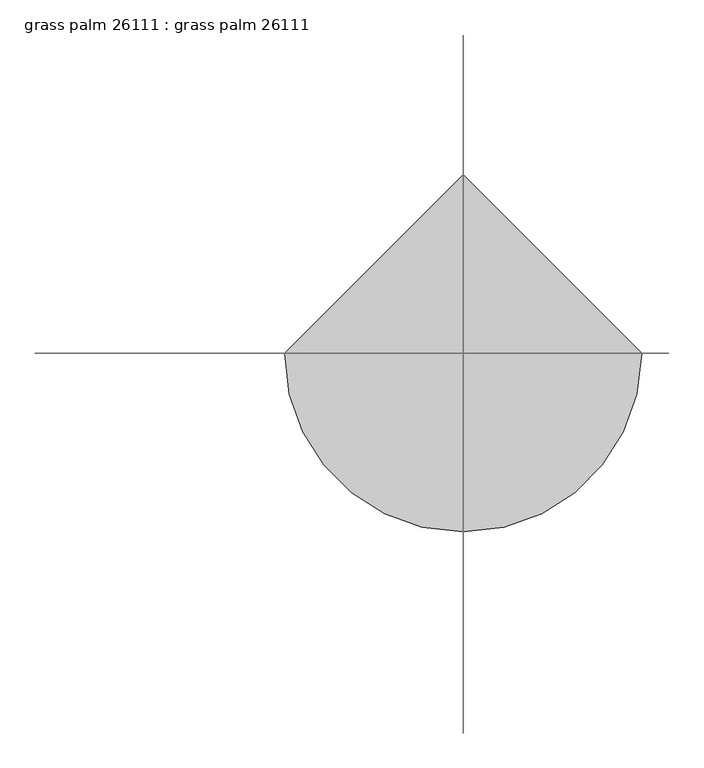
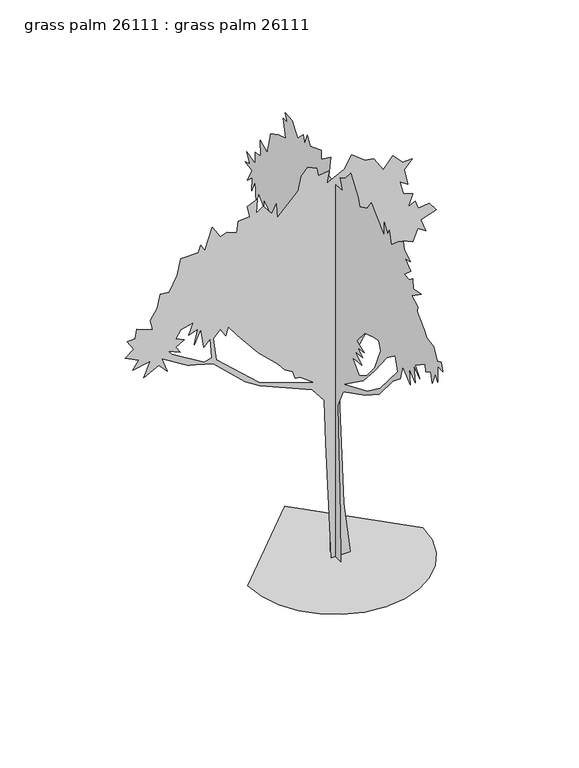
"""IFC4 building model written with IfcOpenShell, lengths in millimetres: proxy geometry, grass palm 26111 : grass palm 26111."""

import ifcopenshell
import ifcopenshell.guid

model = None  # the IFC model being written
_history = None  # IfcOwnerHistory: only IFC2X3 demands one
_inside = {}  # id of a spatial element -> (the spatial element, [elements in it])
_under = {}  # id of a project, library or spatial element -> (it, [spatial elements below it])
_declared = {}  # id of a project -> (the project, [libraries it declares])
_typed = {}  # id of a type object -> (the type object, [elements of that type])
_made_of = {}  # id of a material, layer set ... -> (it, [elements and type objects made of it])


def new_model(schema):
    """Start an empty IFC model of exactly this schema.

    Asked for "IFC4X3", IfcOpenShell would pick the latest addendum, in which some entities
    have other attributes; the version numbers below select the first issue.
    IFC2X3 requires an IfcOwnerHistory on every rooted entity: one is made here for all.
    """
    global model, _history
    if schema == "IFC4X3":
        model = ifcopenshell.file(schema_version=(4, 3, 0, 0))
    else:
        model = ifcopenshell.file(schema=schema)
    _inside.clear()
    _under.clear()
    _declared.clear()
    _typed.clear()
    _made_of.clear()
    _history = None
    if model.schema == "IFC2X3":
        org = make("IfcOrganization", Name="unknown")
        user = make(
            "IfcPersonAndOrganization",
            ThePerson=make("IfcPerson", FamilyName="unknown"),
            TheOrganization=org,
        )
        app = make(
            "IfcApplication",
            ApplicationDeveloper=org,
            Version="unknown",
            ApplicationFullName="unknown",
            ApplicationIdentifier="unknown",
        )
        _history = make(
            "IfcOwnerHistory",
            OwningUser=user,
            OwningApplication=app,
            ChangeAction="ADDED",
            CreationDate=0,
        )
    return model


def make(cls, **values):
    """One entity of the class cls with the attributes given. An attribute that is None is left unset."""
    return model.create_entity(
        cls, **{name: value for name, value in values.items() if value is not None}
    )


def rooted(cls, **values):
    """An entity with a GlobalId (a new one), such as an element, a storey or a relation."""
    return make(cls, GlobalId=ifcopenshell.guid.new(), OwnerHistory=_history, **values)


def si_unit(unit_type, name, prefix=None):
    """IfcSIUnit, for example si_unit("LENGTHUNIT", "METRE", prefix="MILLI")."""
    return make("IfcSIUnit", UnitType=unit_type, Prefix=prefix, Name=name)


def assignment(units):
    """IfcUnitAssignment: the units of a project."""
    return None if units is None else make("IfcUnitAssignment", Units=units)


def point(xyz):
    """IfcCartesianPoint."""
    return None if xyz is None else make("IfcCartesianPoint", Coordinates=xyz)


def direction(xyz):
    """IfcDirection."""
    return None if xyz is None else make("IfcDirection", DirectionRatios=xyz)


def frame(location, z_axis=None, x_axis=None):
    """IfcAxis2Placement3D, a coordinate frame: its origin and axes. An axis left out is left unset."""
    return make(
        "IfcAxis2Placement3D",
        Location=point(location),
        Axis=direction(z_axis),
        RefDirection=direction(x_axis),
    )


def origin():
    """The frame at (0, 0, 0) with its axes left unset."""
    return frame((0.0, 0.0, 0.0))


def place(relative_to, where):
    """IfcLocalPlacement: puts the frame where relative to a parent placement (None: the world)."""
    return make(
        "IfcLocalPlacement", PlacementRelTo=relative_to, RelativePlacement=where
    )


def context(
    kind, dimensions, precision=None, world=None, true_north=None, identifier=None
):
    """IfcGeometricRepresentationContext, for example the 3D "Model" context."""
    return make(
        "IfcGeometricRepresentationContext",
        ContextIdentifier=identifier,
        ContextType=kind,
        CoordinateSpaceDimension=dimensions,
        Precision=precision,
        WorldCoordinateSystem=world,
        TrueNorth=true_north,
    )


def project(units=None, contexts=None):
    """IfcProject with its units and contexts."""
    return rooted(
        "IfcProject",
        Name="project",
        RepresentationContexts=contexts,
        UnitsInContext=assignment(units),
    )


def spatial(cls, under=None, at=None, **own):
    """A site, building, storey or space (cls), placed at a placement, below another one or the project."""
    s = rooted(cls, ObjectPlacement=at, **own)
    if under is not None:
        _under.setdefault(under.id(), (under, []))[1].append(s)
    return s


def point_list(points):
    """IfcCartesianPointList2D or 3D."""
    cls = (
        "IfcCartesianPointList2D" if len(points[0]) == 2 else "IfcCartesianPointList3D"
    )
    return make(cls, CoordList=points)


def triangles(points, corners, closed=None, point_numbers=None):
    """IfcTriangulatedFaceSet: each triangle names its three corners, points numbered from 1."""
    return make(
        "IfcTriangulatedFaceSet",
        Coordinates=point_list(points),
        Closed=closed,
        CoordIndex=corners,
        PnIndex=point_numbers,
    )


def shape(context_of_items, identifier, shape_type, items):
    """IfcShapeRepresentation: the items that make up one representation, for example the "Body"."""
    return make(
        "IfcShapeRepresentation",
        ContextOfItems=context_of_items,
        RepresentationIdentifier=identifier,
        RepresentationType=shape_type,
        Items=items,
    )


def source(mapping_origin, context_of_items, identifier, shape_type, items):
    """IfcRepresentationMap: a shape defined once, which mapped items show again and again."""
    return make(
        "IfcRepresentationMap",
        MappingOrigin=mapping_origin,
        MappedRepresentation=shape(context_of_items, identifier, shape_type, items),
    )


def transform(
    local_origin,
    x_axis=None,
    y_axis=None,
    z_axis=None,
    scale=None,
    scale2=None,
    scale3=None,
    uniform=True,
):
    """IfcCartesianTransformationOperator3D, or its non-uniform kind. x_axis, y_axis, z_axis: its Axis1, 2, 3."""
    if uniform:
        return make(
            "IfcCartesianTransformationOperator3D",
            Axis1=direction(x_axis),
            Axis2=direction(y_axis),
            LocalOrigin=point(local_origin),
            Scale=scale,
            Axis3=direction(z_axis),
        )
    return make(
        "IfcCartesianTransformationOperator3DnonUniform",
        Axis1=direction(x_axis),
        Axis2=direction(y_axis),
        LocalOrigin=point(local_origin),
        Scale=scale,
        Axis3=direction(z_axis),
        Scale2=scale2,
        Scale3=scale3,
    )


def mapped(mapping_source, mapping_target):
    """IfcMappedItem: shows the shape of a source again, moved by a transform."""
    return make(
        "IfcMappedItem", MappingSource=mapping_source, MappingTarget=mapping_target
    )


def made_of(thing, what):
    """Note that an element or type object is made of a material, layer set ...; save() writes the relation."""
    if what is not None:
        _made_of.setdefault(what.id(), (what, []))[1].append(thing)
    return thing


def element(
    cls,
    number,
    at=None,
    inside=None,
    cuts=None,
    type_object=None,
    material=None,
    context=None,
    identifier="Body",
    shape_type=None,
    held_by="IfcProductDefinitionShape",
    body=None,
    shapes=None,
    **own,
):
    """One element of the class cls, such as IfcWall. Its Tag is "e" and its number.

    at: its placement. inside: the storey or other place that contains it. cuts: it is an
    opening in that element (IfcRelVoidsElement). A single representation is given by context,
    identifier, shape_type and body (its items); several are given by shapes. held_by: the class
    of the entity that holds the representations. save() writes the other relations.
    """
    e = rooted(cls, Tag="e%d" % number, ObjectPlacement=at, **own)
    if body is not None:
        shapes = [shape(context, identifier, shape_type, body)]
    if shapes is not None:
        e.Representation = make(held_by, Representations=shapes)
    if inside is not None:
        _inside.setdefault(inside.id(), (inside, []))[1].append(e)
    if cuts is not None:
        rooted(
            "IfcRelVoidsElement", RelatingBuildingElement=cuts, RelatedOpeningElement=e
        )
    if type_object is not None:
        _typed.setdefault(type_object.id(), (type_object, []))[1].append(e)
    return made_of(e, material)


def aggregate(whole, parts):
    """IfcRelAggregates: a whole, such as a stair, and the parts it consists of."""
    return rooted("IfcRelAggregates", RelatingObject=whole, RelatedObjects=parts)


def save(model, path):
    """Write the relations noted so far, then the file.

    IfcRelAggregates (storeys below a building ...), IfcRelContainedInSpatialStructure (elements
    in a storey), IfcRelDefinesByType, IfcRelAssociatesMaterial and IfcRelDeclares: one each for
    every whole, place, type object, material and project.
    """
    for whole, parts in _under.values():
        aggregate(whole, parts)
    for where, things in _inside.values():
        rooted(
            "IfcRelContainedInSpatialStructure",
            RelatedElements=things,
            RelatingStructure=where,
        )
    for kind, things in _typed.values():
        rooted("IfcRelDefinesByType", RelatedObjects=things, RelatingType=kind)
    for what, things in _made_of.values():
        rooted("IfcRelAssociatesMaterial", RelatedObjects=things, RelatingMaterial=what)
    for by, libraries in _declared.values():
        rooted("IfcRelDeclares", RelatingContext=by, RelatedDefinitions=libraries)
    model.write(path)


def grass_palm_26111_grass_palm_26111_ffc4a38a(model_context):
    return source(origin(), model_context, "Body", "Tessellation", [
        triangles([(197.8251161, -0.0004657, 0.0001367), (109.1148514, -0.0002635, 694.5605118), (43.5490633, 0.0002048, 2380.5060047), (409.1686295, 0.0003079, 2962.5546341), (570.4154732, 0.000405, 3409.2137077), (607.6747178, 0.0004576, 3623.4372597), (719.4525244, 0.0004509, 3660.6992294), (654.2481468, 0.0004936, 3781.8063721), (747.397621, 0.0005252, 3949.4717194), (775.3401741, 0.0005007, 3874.9480705), (877.80376, 0.0005308, 4042.6134178), (1008.2098989, 0.0004934, 3977.4115837), (1073.4142765, 0.0005291, 4145.0772217), (1175.8753189, 0.0004934, 4070.5535728), (1110.6734848, 0.0005514, 4247.5407349), (1315.5981857, 0.0005381, 4312.742569), (1222.4487843, 0.0005851, 4433.8244225), (1082.7284609, 0.0006012, 4415.2060822), (1039.2334414, 0.0006388, 4529.6586891), (952.3222492, 0.0006386, 4480.4079163), (1008.2098989, 0.0006732, 4638.7514488), (886.9528381, 0.0007051, 4688.7640938), (840.544479, 0.0007593, 4862.3223953), (943.0055214, 0.0007261, 4797.0952721), (896.4321287, 0.0007914, 5011.3441132), (998.8957146, 0.0008063, 5123.1297318), (877.80376, 0.0008246, 5123.1297318), (747.397621, 0.0008797, 5253.5334), (626.3056664, 0.0008575, 5104.4861023), (503.8725509, 0.0009294, 5301.1072403), (384.1216845, 0.0009523, 5318.7352341), (216.4545022, 0.0010156, 5458.4604263), (113.9921609, 0.0009855, 5290.795079), (-109.5623986, 0.0009889, 5179.0094604), (-81.6183375, 0.0010277, 5337.3532837), (-221.3396873, 0.0010437, 5318.7352341), (-239.9693097, 0.0010769, 5430.5202713), (-361.0610281, 0.0011104, 5486.4005814), (-444.8937381, 0.0010978, 5393.2585922), (-482.1529827, 0.0010527, 5206.9496155), (-752.2819885, 0.0010175, 4927.5242294), (-770.9103573, 0.0010735, 5123.1297318), (-826.8005505, 0.0010516, 5011.3441132), (-938.5783207, 0.0011065, 5151.0698868), (-1031.7252514, 0.0011028, 5085.8680527), (-1013.0943392, 0.0011506, 5272.1514496), (-1143.5030216, 0.0011551, 5216.2711395), (-1115.557925, 0.0011104, 5067.2244232), (-1264.5950489, 0.0011304, 5057.9278976), (-1283.2232723, 0.0010926, 4908.8806), (-1404.3152996, 0.0011236, 4955.4643845), (-1497.4622303, 0.0011301, 4927.5242294), (-1599.9257435, 0.0011911, 5095.1895767), (-1702.389402, 0.0011281, 4806.4170868), (-1748.9628674, 0.0011604, 4899.5590759), (-1786.2220757, 0.0011407, 4806.4170868), (-2009.7751453, 0.0011745, 4806.4170868), (-2056.3486107, 0.0011233, 4592.1932442), (-2158.8122692, 0.0010856, 4396.5624527), (-2279.9041512, 0.0011064, 4405.8842674), (-2317.1635048, 0.0010639, 4228.8971054), (-2410.3102901, 0.00104, 4089.1972023), (-2377.0008408, 0.0009991, 3957.4473953), (-2587.2949814, 0.0010515, 4033.2916031), (-2605.9133217, 0.0010214, 3912.2100403), (-2708.3768349, 0.0010343, 3902.8882256), (-2624.5569511, 0.0009862, 3772.4845573), (-2736.3166992, 0.0009803, 3688.6390938), (-2559.355117, 0.0009282, 3595.4973953), (-2633.853186, 0.0009091, 3483.7117767), (-2410.3102901, 0.000888, 3530.2955612), (-2494.1431091, 0.0008475, 3334.6900589), (-2298.535136, 0.0008458, 3437.1535721), (-2186.7573658, 0.000796, 3316.0464294), (-2261.2733116, 0.0008604, 3511.6772209), (-1928.0074619, 0.0007539, 3305.1500015), (-1586.5374619, 0.000677, 3211.8556961), (-1169.4034029, 0.0005069, 2817.7745178), (-980.3029541, 0.0004448, 2694.5084953), (-299.9587802, 0.0002625, 2401.7378483), (-143.374379, 0.000185, 2203.9150394), (-126.1084725, 2.08e-05, 1609.6107628), (-53.6737587, -0.0004278, 0.0001367), (-1497.4622303, 0.0008957, 3651.4027039), (-1422.9462845, 0.000854, 3539.6173759), (-1395.0011879, 0.0008802, 3651.4027039), (-1273.9091606, 0.0008189, 3493.0335915), (-1002.0681953, 0.0003602, 3156.4073364), (-744.7432772, 0.0005791, 2905.2014488), (-659.9860233, 0.000538, 2801.1377426), (-556.6715083, 0.0005054, 2738.5520279), (-519.4122637, 0.0004719, 2636.0885147), (-454.2079225, 0.0004596, 2626.7667), (-267.9141337, 0.0003934, 2487.0438332), (-995.0831566, 0.0005747, 2749.8295372), (-1549.5677708, 0.0007954, 3253.765638), (-1590.6116318, 0.0008844, 3558.2354256), (-2019.0918732, 0.0008854, 3520.9737465), (-2074.9794502, 0.0009166, 3604.8192101), (-1963.20168, 0.0009175, 3670.0207535), (-2074.9794502, 0.0009495, 3725.9007729), (-2009.7751453, 0.0009676, 3828.3645767), (-1851.4239098, 0.0009538, 3865.6262558), (-1907.3141029, 0.0009217, 3716.604538), (-1791.7262455, 0.0009145, 3754.1964294), (-1838.0305412, 0.0008682, 3558.4641907), (-1748.9628674, 0.0009054, 3744.5444023), (-1711.7036591, 0.0008288, 3483.7117767), (-1627.8708401, 0.000839, 3567.5572403), (-1608.65835, 0.0007633, 3299.7651558), (-1708.7927902, 0.0007706, 3271.2916031), (-2130.8671726, 0.0009048, 3530.2955612), (-2177.4431087, 0.000927, 3586.1755806), (0.0001009, -125.9822357, 0.0001592), (6.27e-05, -114.0061317, 632.7801258), (3.21e-05, -52.0852428, 2115.3046051), (1.35e-05, -175.1038104, 2373.6836014), (-6.14e-05, -671.5328476, 2630.4243256), (-0.0001496, -990.5162842, 2836.0117767), (-0.0001562, -1298.9586491, 3200.2479744), (-0.0001816, -1467.3098557, 3334.6900589), (-0.00019, -1523.1974327, 3539.6173759), (-0.0002153, -1690.8629253, 3390.5700783), (-0.0002111, -1662.9202995, 3595.4973953), (-0.0002322, -1802.6406956, 3483.7373566), (-0.0002266, -1765.3814873, 3707.2827232), (-0.0002477, -1905.101738, 3604.8192101), (-0.0002322, -1802.6406956, 3725.9007729), (-0.000266, -2026.196236, 3874.9480705), (-0.0002688, -2044.8246048, 3781.8063721), (-0.0002843, -2147.2882633, 3837.6863914), (-0.0002899, -2184.5450008, 3707.2827232), (-0.0002997, -2249.7493057, 3874.9480705), (-0.0003096, -2314.9536106, 3800.4244217), (-0.0003096, -2314.9536106, 4023.9697884), (-0.0003265, -2426.7289101, 4014.6735535), (-0.0003208, -2389.4721725, 4126.4335922), (-0.0003068, -2296.3227711, 4079.8753876), (-0.0002955, -2221.8042091, 4238.2189201), (-0.0002716, -2063.4555897, 4266.1590752), (-0.0002632, -2007.5653965, 4340.6824333), (-0.0002792, -1849.2141609, 4489.729731), (-0.0002806, -1858.5282726, 4564.2280907), (-0.0002609, -1728.1221336, 4638.7514488), (-0.0002933, -1942.3609463, 4787.7987465), (-0.0002652, -1756.0672302, 4750.5370674), (-0.0002638, -1746.7531185, 4880.9404449), (-0.0002525, -1672.2345566, 4825.0607162), (-0.0002356, -1560.4567863, 4834.3569511), (-0.0002567, -1700.177037, 4955.4643845), (-0.0002384, -1579.0876259, 5057.9278976), (-0.0002553, -1690.8629253, 5085.8680527), (-0.0002342, -1551.1425293, 5169.6879364), (-0.0002314, -1532.5116898, 5262.854924), (-0.0002145, -1420.7339195, 5197.6530899), (-0.0001906, -1262.3826839, 5057.9278976), (-0.0001836, -1215.8092186, 5225.5932449), (-0.000178, -1178.5499376, 5151.0698868), (-0.0002067, -1104.0339191, 5272.1514496), (-0.0001667, -1104.0339191, 5085.8680527), (-0.0001811, -934.8191025, 5242.9666031), (-0.0001617, -805.9598167, 5355.9969131), (-0.0001497, -726.4933737, 5236.9472031), (-0.0001237, -554.4617231, 5151.0698868), (-0.0001181, -517.2024785, 5253.5334), (-9.28e-05, -349.5370585, 5486.4005814), (-7.45e-05, -228.4440684, 5346.6748077), (-5.62e-05, -107.3520956, 5281.4729736), (-6.46e-05, -163.2409807, 5132.4512558), (-4.21e-05, -14.2045188, 5123.1297318), (-1.82e-05, 144.1465339, 5151.0698868), (-2.38e-05, 106.8877798, 5430.5202713), (7.1e-06, 311.8129804, 5281.4729736), (7.1e-06, 311.8129804, 5402.5551178), (4.51e-05, 563.311074, 5309.4131287), (5.49e-05, 628.5154152, 5421.1987473), (6.48e-05, 693.7172493, 5262.854924), (6.9e-05, 721.6623459, 5365.3184372), (8.73e-05, 842.7543005, 5244.2112946), (9.71e-05, 907.9586054, 5309.4131287), (0.000107, 973.1604395, 5411.8766418), (9.09e-05, 1131.5116751, 5421.1987473), (0.0001238, 1084.9382097, 5318.7352341), (0.0001369, 1171.5319067, 5326.1010635), (0.0001281, 1112.8833063, 5085.8680527), (0.0001548, 1289.862838, 5020.6662186), (0.0001793, 1452.3822784, 4938.471817), (0.0001914, 1532.0468925, 4629.4296341), (0.0002153, 1690.3981281, 4703.9532829), (0.0002139, 1681.0838711, 4489.729731), (0.0002321, 1802.1758984, 4471.0861015), (0.0002321, 1802.1758984, 4312.742569), (0.0002617, 1997.7863422, 4359.3007736), (0.0002506, 1924.1873463, 4240.2763527), (0.0002671, 2033.8797787, 4204.1576271), (0.0002434, 1876.6944603, 4173.017086), (0.0002603, 1988.4722305, 3977.4115837), (0.000242, 1867.3802032, 4079.8753876), (0.0002448, 1886.008572, 3893.5664108), (0.0002321, 1802.1758984, 4070.5535728), (0.0002293, 1783.5475296, 3791.102607), (0.0002209, 1727.6573364, 3949.4717194), (0.000204, 1615.8795662, 3837.6863914), (0.000204, 1615.8795662, 3940.1499046), (0.0001974, 1307.620039, 3736.3911209), (0.0001385, 917.2727898, 3623.4372597), (0.0001194, 790.5928768, 3229.1531868), (0.0001184, 784.0523603, 3133.6235527), (0.0001019, 675.0888805, 3064.5609077), (0.0001273, 842.7543005, 2934.1575302), (0.0001104, 730.9765303, 2971.4192093), (0.0001532, 749.6048264, 2775.813707), (0.0001377, 647.143784, 2906.2173752), (0.0001349, 628.5154152, 2673.3501938), (0.0001307, 600.5703549, 2775.813707), (0.0001264, 572.6252584, 2673.3501938), (0.0001194, 526.0518293, 2841.0155411), (0.0001152, 498.1067327, 2682.6467194), (0.0001124, 479.478364, 2608.1483597), (0.0001067, 442.2191194, 2738.5520279), (9.69e-05, 377.0147781, 2654.7065643), (7.78e-05, 250.6550855, 2492.941729), (2.45e-05, 161.9890223, 2108.946999), (9.68e-05, 111.8545007, 1061.9156324), (0.0001375, 116.2017099, 0.0001159), (-9.51e-05, -630.0470804, 2801.0107155), (-0.0001338, -885.9978092, 3096.8699821), (-0.0001753, -1160.7521868, 3441.0905411), (-0.0002047, -1355.5320854, 3586.1755806), (-0.0002131, -1411.4196625, 3399.891893), (-0.0001538, -1018.750898, 2931.8969124), (-0.0001089, -721.0450871, 2712.8219124), (-2.89e-05, -191.1855686, 2487.0438332), (-6.83e-05, -451.9981009, 2980.7157349), (-8.93e-05, -591.7210041, 2990.0375496), (-6.83e-05, -451.9981009, 3092.5010628), (-9.36e-05, -619.6661007, 3111.1446922), (-7.67e-05, -507.7485861, 3183.8393829), (-9.92e-05, -656.9227655, 3204.2863907), (-7.39e-05, -489.2573819, 3269.4882248), (-0.0001003, -664.5148893, 3478.2763527), (-0.0001315, -871.1641943, 3548.9391907), (-0.0001484, -982.9419645, 3567.5572403), (-0.0001546, -1023.6937649, 3456.6608116), (-0.0001342, -889.0838854, 3136.1382248), (-0.0001091, -722.497978, 2934.7415062), (-8.09e-05, -535.8308109, 2813.0500969), (-5.98e-05, -396.1104876, 2971.4192093), (-1140.1273556, 0.0, 0.0001367), (-1109.9876982, -261.2415577, 0.0001834), (-1024.1458448, -501.1521864, 0.0002263), (-889.4750679, -712.8535812, 0.0002641), (-712.8535812, -889.4750679, 0.0002957), (-501.1496429, -1024.1458448, 0.0), (-261.2415577, -1109.9876982, 1.53e-05), (6.77e-05, -1140.1273556, 2.07e-05), (261.2415577, -1109.9876982, 1.53e-05), (501.1521864, -1024.1458448, 0.0), (712.8535812, -889.4750679, 0.0002957), (889.4750679, -712.8535812, 0.0002641), (1024.1458448, -501.1496429, 0.0002263), (1109.9876982, -261.2415577, 0.0001834), (1140.1273556, 9.97e-05, 0.0001367), (-0.0001476, 1140.1273556, 0.0002526)], [[95, 110, 96], [86, 3, 87], [87, 3, 88], [88, 3, 89], [106, 105, 107], [89, 3, 90], [90, 3, 91], [74, 73, 75], [42, 41, 43], [14, 13, 15], [98, 113, 99], [72, 71, 73], [96, 110, 97], [110, 109, 97], [70, 69, 71], [24, 23, 25], [26, 25, 27], [85, 84, 86], [55, 54, 56], [53, 52, 54], [104, 103, 105], [10, 9, 11], [108, 107, 109], [100, 99, 101], [46, 45, 47], [47, 45, 48], [66, 65, 67], [68, 67, 69], [16, 15, 17], [17, 15, 18], [35, 34, 36], [73, 71, 75], [64, 63, 65], [7, 6, 8], [3, 86, 4], [19, 18, 20], [32, 31, 33], [1, 83, 2], [83, 82, 2], [2, 82, 3], [82, 81, 3], [28, 27, 29], [12, 11, 13], [81, 80, 3], [4, 86, 5], [5, 86, 6], [21, 20, 22], [44, 43, 45], [27, 25, 29], [25, 23, 29], [60, 59, 61], [99, 113, 101], [49, 48, 50], [57, 56, 58], [6, 86, 8], [38, 37, 39], [37, 36, 39], [39, 36, 40], [36, 34, 40], [65, 63, 67], [67, 63, 69], [69, 63, 71], [71, 63, 75], [92, 91, 93], [91, 3, 93], [93, 3, 94], [3, 80, 94], [80, 79, 94], [94, 79, 95], [79, 78, 95], [95, 78, 110], [78, 77, 110], [110, 77, 111], [77, 76, 111], [111, 76, 112], [76, 75, 112], [112, 75, 113], [75, 63, 113], [113, 63, 101], [101, 63, 102], [97, 109, 84], [109, 107, 84], [8, 86, 9], [63, 62, 102], [62, 61, 102], [61, 59, 102], [102, 59, 103], [59, 58, 103], [58, 56, 103], [56, 54, 103], [18, 15, 20], [15, 13, 20], [13, 11, 20], [54, 52, 103], [52, 51, 103], [51, 50, 103], [103, 50, 105], [105, 50, 107], [107, 50, 84], [84, 50, 86], [86, 50, 9], [50, 48, 9], [48, 45, 9], [40, 34, 41], [30, 29, 31], [31, 29, 33], [33, 29, 34], [11, 9, 20], [29, 23, 34], [23, 22, 34], [34, 22, 41], [22, 20, 41], [20, 9, 41], [9, 45, 41], [45, 43, 41], [226, 245, 246], [245, 226, 227], [233, 116, 117], [126, 127, 128], [209, 210, 211], [198, 199, 200], [213, 214, 215], [196, 197, 198], [226, 246, 247], [200, 201, 202], [144, 145, 146], [238, 239, 240], [194, 195, 196], [218, 219, 220], [215, 216, 217], [158, 159, 160], [211, 212, 213], [245, 227, 228], [244, 245, 228], [131, 132, 133], [236, 237, 238], [234, 235, 236], [122, 123, 124], [133, 134, 135], [124, 125, 126], [156, 157, 158], [233, 226, 247], [192, 193, 194], [202, 203, 204], [151, 152, 153], [171, 172, 173], [175, 176, 177], [233, 117, 118], [232, 233, 118], [232, 118, 119], [231, 232, 119], [231, 119, 120], [230, 231, 120], [230, 120, 121], [217, 218, 220], [230, 121, 122], [229, 230, 122], [146, 147, 148], [177, 178, 179], [181, 182, 183], [188, 189, 190], [135, 136, 137], [135, 137, 138], [213, 215, 217], [173, 174, 175], [153, 154, 155], [183, 184, 185], [129, 130, 131], [165, 166, 167], [149, 150, 151], [161, 162, 163], [180, 181, 183], [192, 194, 196], [225, 114, 115], [224, 225, 115], [224, 115, 116], [223, 224, 116], [156, 158, 160], [233, 247, 248], [180, 183, 185], [179, 180, 185], [209, 211, 213], [167, 168, 169], [165, 167, 169], [164, 165, 169], [190, 191, 192], [248, 234, 236], [222, 223, 116], [222, 116, 233], [196, 198, 200], [222, 233, 248], [221, 222, 248], [220, 221, 248], [142, 143, 144], [217, 220, 248], [192, 196, 200], [151, 153, 155], [151, 155, 156], [149, 151, 156], [243, 244, 228], [243, 228, 229], [144, 146, 148], [144, 148, 149], [217, 248, 236], [138, 139, 140], [207, 208, 209], [200, 202, 204], [192, 200, 204], [190, 192, 204], [188, 190, 204], [188, 204, 205], [188, 205, 206], [209, 213, 217], [209, 217, 236], [209, 236, 238], [209, 238, 240], [207, 209, 240], [206, 207, 240], [206, 240, 241], [188, 206, 241], [187, 188, 241], [186, 187, 241], [185, 186, 241], [179, 185, 241], [177, 179, 241], [175, 177, 241], [173, 175, 241], [171, 173, 241], [170, 171, 241], [169, 170, 241], [164, 169, 241], [164, 241, 242], [164, 242, 243], [163, 164, 243], [161, 163, 243], [160, 161, 243], [160, 243, 229], [156, 160, 229], [149, 156, 229], [144, 149, 229], [142, 144, 229], [141, 142, 229], [141, 229, 122], [141, 122, 124], [141, 124, 126], [141, 126, 128], [141, 128, 129], [140, 141, 129], [138, 140, 129], [138, 129, 131], [138, 131, 133], [138, 133, 135], [263, 264, 249], [262, 263, 249], [262, 249, 250], [261, 262, 250], [261, 250, 251], [261, 251, 252], [260, 261, 252], [259, 260, 252], [259, 252, 253], [259, 253, 254], [259, 254, 255], [259, 255, 256], [259, 256, 257], [259, 257, 258]], closed=False),
    ])


if __name__ == "__main__":
    model = new_model("IFC4")
    model_context = context("Model", 3, world=origin())
    ifc_project = project(units=[si_unit("LENGTHUNIT", "METRE", prefix="MILLI")], contexts=[model_context])
    site = spatial("IfcSite", under=ifc_project)
    building = spatial("IfcBuilding", under=site)
    placement = place(None, origin())
    grass_palm_26111_grass_palm_26111_shape = grass_palm_26111_grass_palm_26111_ffc4a38a(model_context)
    element("IfcBuildingElementProxy", 1, Name="grass palm 26111 : grass palm 26111", ObjectType="grass palm 26111 : grass palm 26111", at=placement, inside=building, context=model_context, shape_type="MappedRepresentation", body=[
        mapped(grass_palm_26111_grass_palm_26111_shape, transform((0.0, 0.0, 0.0), x_axis=(1.0, 0.0, 0.0), y_axis=(0.0, 1.0, 0.0), z_axis=(0.0, 0.0, 1.0))),
    ])
    save(model, "model.ifc")

# Revit data of these elements
# Type "grass palm 26111 : grass palm 26111"
#   built-in parameter 1005195 = "RPC-16-FXGK-2WG0-PNFG-U000-ST1L-LVER-AU"
#   Height = 0
